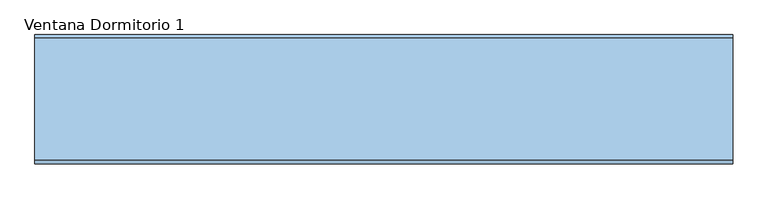
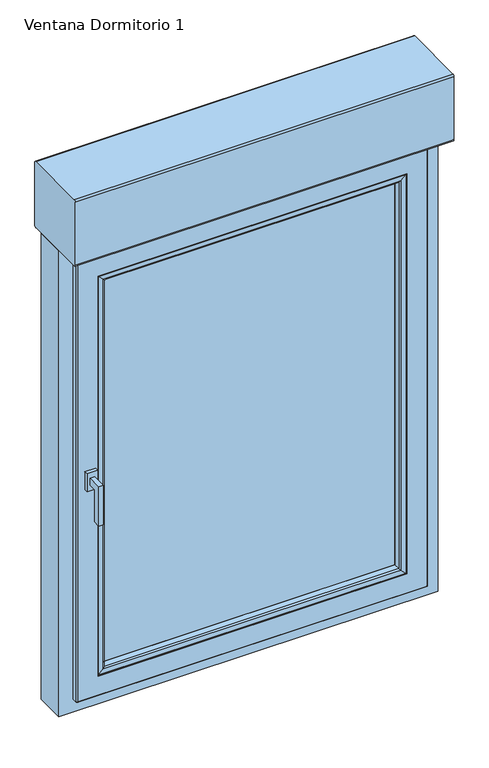
"""IFC4 building model written with IfcOpenShell, lengths in millimetres: window geometry, 2019_ES_Ventana_Replus_re80pvc301_10100_box_1-Hoja_con-Compacto : Ventana Dormitorio 1."""

from ifc_helpers import new_model, si_unit, point, frame, frame_2d, origin, place, context, project, spatial, polyline, circle_curve, ellipse_curve, trimmed, segment, composite_curve, outline, extrude, source, transform, mapped, element, save
from ifc_brep_helpers import plane_surface, cylinder_surface, advanced_brep


def ventana_dormitorio_1_e636b9de(model_context):
    return source(origin(), model_context, "Body", "SolidModel", [
        extrude(outline(composite_curve([segment(polyline([(55.0, 2110.0), (-120.0, 2110.0)]), True, "CONTINUOUS"), segment(trimmed(circle_curve(frame_2d((-120.0, 2115.0)), 5.0), [point((-120.0, 2110.0))], [point((-125.0, 2115.0))], False, "CARTESIAN"), True, "CONTINUOUS"), segment(polyline([(-125.0, 2115.0), (-125.0, 2290.0)]), True, "CONTINUOUS"), segment(trimmed(circle_curve(frame_2d((-120.0, 2290.0)), 5.0), [point((-125.0, 2290.0))], [point((-120.0, 2295.0))], False, "CARTESIAN"), True, "CONTINUOUS"), segment(polyline([(-120.0, 2295.0), (55.0, 2295.0)]), True, "CONTINUOUS"), segment(trimmed(circle_curve(frame_2d((55.0, 2290.0)), 5.0), [point((55.0, 2295.0))], [point((60.0, 2290.0))], False, "CARTESIAN"), True, "CONTINUOUS"), segment(polyline([(60.0, 2290.0), (60.0, 2115.0)]), True, "CONTINUOUS"), segment(trimmed(circle_curve(frame_2d((55.0, 2115.0)), 5.0), [point((60.0, 2115.0))], [point((55.0, 2110.0))], False, "CARTESIAN"), True, "CONTINUOUS")], self_intersect=False)), frame((-500.0, 0.0, 0.0), z_axis=(1.0, 0.0, 0.0), x_axis=(0.0, 1.0, 0.0)), (0.0, 0.0, 1.0), 1000.0),
        extrude(outline(polyline([(-78.4999991, 1470.0), (-78.4999991, 1450.0), (-98.4999991, 1450.0), (-98.4999991, 1360.0), (-118.4999991, 1360.0), (-118.4999991, 1470.0), (-78.4999991, 1470.0)])), frame((-434.1999993, 0.0, 0.0), z_axis=(1.0, 0.0, 0.0), x_axis=(0.0, 1.0, 0.0)), (0.0, 0.0, 1.0), 12.0),
        extrude(outline(polyline([(-413.9687607, -78.4999991), (-442.4312378, -78.4999991), (-442.4312378, -68.4999991), (-413.9687607, -68.4999991), (-413.9687607, -78.4999991)])), frame((0.0, 0.0, 1435.217127), z_axis=(0.0, 0.0, 1.0), x_axis=(1.0, 0.0, 0.0)), (0.0, 0.0, 1.0), 49.565746),
        extrude(outline(polyline([(2007.2, 397.1999993), (2007.2, -397.1999993), (909.8, -397.1999993), (909.8, 397.1999993), (2007.2, 397.1999993)]), holes=[polyline([(917.8, 389.1999993), (917.8, -389.1999993), (1999.2, -389.1999993), (1999.2, 389.1999993), (917.8, 389.1999993)])]), frame((0.0, -26.9999999, 0.0), z_axis=(0.0, 1.0, 0.0), x_axis=(0.0, 0.0, 1.0)), (0.0, 0.0, 1.0), 16.0),
        extrude(outline(polyline([(2007.1868066, 397.1868058), (2007.1868066, -397.1868058), (909.8131934, -397.1868058), (909.8131934, 397.1868058), (2007.1868066, 397.1868058)]), holes=[polyline([(917.8, 389.1999993), (917.8, -389.1999993), (1999.2, -389.1999993), (1999.2, 389.1999993), (917.8, 389.1999993)])]), frame((0.0, -47.0000001, 0.0), z_axis=(0.0, 1.0, 0.0), x_axis=(0.0, 0.0, 1.0)), (0.0, 0.0, 1.0), 16.0),
        extrude(outline(polyline([(397.1999993, -6.9999997), (397.1999993, -10.9999999), (-397.1999993, -10.9999999), (-397.1999993, -6.9999997), (397.1999993, -6.9999997)])), frame((0.0, 0.0, 903.7946451), z_axis=(0.0, 0.0, 1.0), x_axis=(1.0, 0.0, 0.0)), (0.0, 0.0, 1.0), 1109.4053549),
        extrude(outline(polyline([(397.1999993, -26.9999999), (397.1999993, -31.0000001), (-397.1999993, -31.0000001), (-397.1999993, -26.9999999), (397.1999993, -26.9999999)])), frame((0.0, 0.0, 903.7946451), z_axis=(0.0, 0.0, 1.0), x_axis=(1.0, 0.0, 0.0)), (0.0, 0.0, 1.0), 1109.4053549),
        extrude(outline(polyline([(397.1999993, -47.0000001), (397.1999993, -51.0000003), (-397.1999993, -51.0000003), (-397.1999993, -47.0000001), (397.1999993, -47.0000001)])), frame((0.0, 0.0, 903.7946451), z_axis=(0.0, 0.0, 1.0), x_axis=(1.0, 0.0, 0.0)), (0.0, 0.0, 1.0), 1109.4053549),
        advanced_brep(
        [(387.2913171, 9.2764571, 1997.2913178), (390.1890946, 11.5, 2000.1890953), (390.1890946, 11.5, 919.8109047), (387.2913171, 9.2764571, 922.7086822), (430.1999993, 11.5, 879.8), (-430.1999993, 11.5, 879.8), (-430.1999993, 11.5, 2040.2), (430.1999993, 11.5, 2040.2), (-390.1890946, 11.5, 2000.1890953), (-390.1890946, 11.5, 919.8109047), (-387.2913171, 9.2764571, 922.7086822), (384.1757968, -2.3508228, 1994.1757976), (384.1757968, -2.3508228, 925.8242024), (-384.1757968, -2.3508228, 925.8242024), (384.6739305, -3.0000033, 1994.6739313), (384.6739305, -3.0000033, 925.3260687), (-384.6739305, -3.0000033, 925.3260687), (391.1999993, -3.0000033, 2001.2), (-391.1999993, -3.0000033, 2001.2), (-391.1999993, -3.0000033, 918.8), (391.1999993, -3.0000033, 918.8), (-384.6739305, -3.0000033, 1994.6739313), (391.1999993, -6.9999997, 2001.2), (391.1999993, -6.9999997, 918.8), (-391.1999993, -6.9999997, 918.8), (411.8162192, -6.9999997, 2021.8162199), (-411.8162192, -6.9999997, 2021.8162199), (-411.8162192, -6.9999997, 898.1837801), (411.8162192, -6.9999997, 898.1837801), (-391.1999993, -6.9999997, 2001.2), (409.1999993, -25.6153717, 2019.2), (409.1999993, -25.6153717, 900.8), (-409.1999993, -25.6153717, 900.8), (409.1999993, -56.4999995, 2019.2), (409.1999993, -56.4999995, 900.8), (-409.1999993, -56.4999995, 900.8), (-409.1999993, -56.4999995, 2019.2), (397.1999993, -56.4999995, 2007.2), (-397.1999993, -56.4999995, 2007.2), (-397.1999993, -56.4999995, 912.8), (397.1999993, -56.4999995, 912.8), (397.1999993, -51.0000003, 2007.2), (397.1999993, -51.0000003, 912.8), (-397.1999993, -51.0000003, 912.8), (-397.1999993, -51.0000003, 2007.2), (386.007687, -51.0000003, 1996.0076877), (-386.007687, -51.0000003, 1996.0076877), (-386.007687, -51.0000003, 923.9923123), (386.007687, -51.0000003, 923.9923123), (385.4940999, -51.6693201, 1995.4941006), (385.4940999, -51.6693201, 924.5058994), (-385.4940999, -51.6693201, 924.5058994), (388.8993918, -64.3780426, 1998.8993925), (388.8993918, -64.3780426, 921.1006075), (-388.8993918, -64.3780426, 921.1006075), (392.6234971, -67.3403297, 2002.6234978), (392.6234971, -67.3403297, 917.3765022), (-392.6234971, -67.3403297, 917.3765022), (405.6488427, -67.7951848, 2015.6488434), (405.6488427, -67.7951848, 904.3511566), (-405.6488427, -67.7951848, 904.3511566), (406.1999993, -67.2629391, 2016.2), (406.1999993, -67.2629391, 903.8), (-406.1999993, -67.2629391, 903.8), (407.4370593, -68.4999991, 2017.43706), (407.4370593, -68.4999991, 902.56294), (-407.4370593, -68.4999991, 902.56294), (460.1999993, -68.4999991, 2070.2), (-460.1999993, -68.4999991, 2070.2), (-460.1999993, -68.4999991, 849.8), (460.1999993, -68.4999991, 849.8), (-407.4370593, -68.4999991, 2017.43706), (463.1999993, -65.4999991, 2073.2), (463.1999993, -65.4999991, 846.8), (-463.1999993, -65.4999991, 846.8), (463.1999993, -50.0, 2073.2), (463.1999993, -50.0, 846.8), (-463.1999993, -50.0, 846.8), (-463.1999993, -50.0, 2073.2), (443.1999993, -50.0, 2053.2), (-443.1999993, -50.0, 2053.2), (-443.1999993, -50.0, 866.8), (443.1999993, -50.0, 866.8), (443.1999993, -11.9999991, 866.8), (443.1999993, -11.9999991, 2053.2), (-443.1999993, -11.9999991, 866.8), (-443.1999993, -11.9999991, 2053.2), (430.1999993, -11.9999991, 2040.2), (-430.1999993, -11.9999991, 2040.2), (-430.1999993, -11.9999991, 879.8), (430.1999993, -11.9999991, 879.8), (-387.2913171, 9.2764571, 1997.2913178), (-384.1757968, -2.3508228, 1994.1757976), (-409.1999993, -25.6153717, 2019.2), (-385.4940999, -51.6693201, 1995.4941006), (-388.8993918, -64.3780426, 1998.8993925), (-392.6234971, -67.3403297, 2002.6234978), (-405.6488427, -67.7951848, 2015.6488434), (-406.1999993, -67.2629391, 2016.2), (-463.1999993, -65.4999991, 2073.2)],
        [
            (0, 1, ellipse_curve(frame((390.1890946, 8.5, 2000.1890953), z_axis=(0.7071067811865475, 0.0, -0.7071067811865475), x_axis=(0.7071067811865474, 0.0, 0.7071067811865476)), 4.2426407, 3.0)),
            (1, 2),
            (2, 3, ellipse_curve(frame((390.1890946, 8.5, 919.8109047), z_axis=(0.7071067811865475, 0.0, 0.7071067811865475), x_axis=(-0.7071067811865474, 0.0, 0.7071067811865476)), 4.2426407, 3.0)),
            (3, 0),
            (4, 5),
            (5, 6),
            (6, 7),
            (7, 4),
            (1, 8),
            (8, 9),
            (9, 2),
            (9, 10, ellipse_curve(frame((-390.1890946, 8.5, 919.8109047), z_axis=(0.7071067811865475, 0.0, -0.7071067811865475), x_axis=(0.7071067811865476, 0.0, 0.7071067811865474)), 4.2426407, 3.0)),
            (10, 3),
            (11, 0),
            (3, 12),
            (12, 11),
            (10, 13),
            (13, 12),
            (14, 11, ellipse_curve(frame((384.6739305, -2.4842973, 1994.6739313), z_axis=(0.7071067811865475, 0.0, -0.7071067811865475), x_axis=(0.7071067811865474, 0.0, 0.7071067811865476)), 0.7293184, 0.515706)),
            (12, 15, ellipse_curve(frame((384.6739305, -2.4842973, 925.3260687), z_axis=(0.7071067811865475, 0.0, 0.7071067811865475), x_axis=(-0.7071067811865474, 0.0, 0.7071067811865476)), 0.7293184, 0.515706)),
            (15, 14),
            (13, 16, ellipse_curve(frame((-384.6739305, -2.4842973, 925.3260687), z_axis=(0.7071067811865475, 0.0, -0.7071067811865475), x_axis=(0.7071067811865476, 0.0, 0.7071067811865474)), 0.7293184, 0.515706)),
            (16, 15),
            (17, 18),
            (18, 19),
            (19, 20),
            (20, 17),
            (16, 21),
            (21, 14),
            (22, 17),
            (20, 23),
            (23, 22),
            (19, 24),
            (24, 23),
            (25, 26),
            (26, 27),
            (27, 28),
            (28, 25),
            (24, 29),
            (29, 22),
            (30, 25),
            (28, 31),
            (31, 30),
            (27, 32),
            (32, 31),
            (33, 30),
            (31, 34),
            (34, 33),
            (32, 35),
            (35, 34),
            (35, 36),
            (36, 33),
            (37, 38),
            (38, 39),
            (39, 40),
            (40, 37),
            (41, 37),
            (40, 42),
            (42, 41),
            (39, 43),
            (43, 42),
            (43, 44),
            (44, 41),
            (45, 46),
            (46, 47),
            (47, 48),
            (48, 45),
            (49, 45, ellipse_curve(frame((386.007687, -51.5317048, 1996.0076877), z_axis=(0.7071067811865475, 0.0, -0.7071067811865475), x_axis=(0.7071067811865474, 0.0, 0.7071067811865476)), 0.7519437, 0.5317045)),
            (48, 50, ellipse_curve(frame((386.007687, -51.5317048, 923.9923123), z_axis=(0.7071067811865475, 0.0, 0.7071067811865475), x_axis=(-0.7071067811865474, 0.0, 0.7071067811865476)), 0.7519437, 0.5317045)),
            (50, 49),
            (47, 51, ellipse_curve(frame((-386.007687, -51.5317048, 923.9923123), z_axis=(0.7071067811865475, 0.0, -0.7071067811865475), x_axis=(0.7071067811865476, 0.0, 0.7071067811865474)), 0.7519437, 0.5317045)),
            (51, 50),
            (52, 49),
            (50, 53),
            (53, 52),
            (51, 54),
            (54, 53),
            (55, 52, ellipse_curve(frame((392.7630951, -63.3427664, 2002.7630958), z_axis=(0.7071067811865475, 0.0, -0.7071067811865475), x_axis=(0.7071067811865474, 0.0, 0.7071067811865476)), 5.6568542, 4.0)),
            (53, 56, ellipse_curve(frame((392.7630951, -63.3427664, 917.2369042), z_axis=(0.7071067811865475, 0.0, 0.7071067811865475), x_axis=(-0.7071067811865474, 0.0, 0.7071067811865476)), 5.6568542, 4.0)),
            (56, 55),
            (54, 57, ellipse_curve(frame((-392.7630951, -63.3427664, 917.2369042), z_axis=(0.7071067811865475, 0.0, -0.7071067811865475), x_axis=(0.7071067811865476, 0.0, 0.7071067811865474)), 5.6568542, 4.0)),
            (57, 56),
            (58, 55),
            (56, 59),
            (59, 58),
            (57, 60),
            (60, 59),
            (61, 58, ellipse_curve(frame((405.6674291, -67.2629391, 2015.6674299), z_axis=(0.7071067811865475, 0.0, -0.7071067811865475), x_axis=(0.7071067811865474, 0.0, 0.7071067811865476)), 0.7531679, 0.5325701)),
            (59, 62, ellipse_curve(frame((405.6674291, -67.2629391, 904.3325701), z_axis=(0.7071067811865475, 0.0, 0.7071067811865475), x_axis=(-0.7071067811865474, 0.0, 0.7071067811865476)), 0.7531679, 0.5325701)),
            (62, 61),
            (60, 63, ellipse_curve(frame((-405.6674291, -67.2629391, 904.3325701), z_axis=(0.7071067811865475, 0.0, -0.7071067811865475), x_axis=(0.7071067811865476, 0.0, 0.7071067811865474)), 0.7531679, 0.5325701)),
            (63, 62),
            (64, 61, ellipse_curve(frame((407.4370593, -67.2629391, 2017.43706), z_axis=(0.7071067811865475, 0.0, -0.7071067811865475), x_axis=(0.7071067811865474, 0.0, 0.7071067811865476)), 1.7494671, 1.23706)),
            (62, 65, ellipse_curve(frame((407.4370593, -67.2629391, 902.56294), z_axis=(0.7071067811865475, 0.0, 0.7071067811865475), x_axis=(-0.7071067811865474, 0.0, 0.7071067811865476)), 1.7494671, 1.23706)),
            (65, 64),
            (63, 66, ellipse_curve(frame((-407.4370593, -67.2629391, 902.56294), z_axis=(0.7071067811865475, 0.0, -0.7071067811865475), x_axis=(0.7071067811865476, 0.0, 0.7071067811865474)), 1.7494671, 1.23706)),
            (66, 65),
            (67, 68),
            (68, 69),
            (69, 70),
            (70, 67),
            (66, 71),
            (71, 64),
            (72, 67, ellipse_curve(frame((460.1999993, -65.4999991, 2070.2), z_axis=(0.7071067811865475, 0.0, -0.7071067811865475), x_axis=(0.7071067811865474, 0.0, 0.7071067811865476)), 4.2426407, 3.0)),
            (70, 73, ellipse_curve(frame((460.1999993, -65.4999991, 849.8), z_axis=(0.7071067811865475, 0.0, 0.7071067811865475), x_axis=(-0.7071067811865474, 0.0, 0.7071067811865476)), 4.2426407, 3.0)),
            (73, 72),
            (69, 74, ellipse_curve(frame((-460.1999993, -65.4999991, 849.8), z_axis=(0.7071067811865475, 0.0, -0.7071067811865475), x_axis=(0.7071067811865476, 0.0, 0.7071067811865474)), 4.2426407, 3.0)),
            (74, 73),
            (75, 72),
            (73, 76),
            (76, 75),
            (74, 77),
            (77, 76),
            (77, 78),
            (78, 75),
            (79, 80),
            (80, 81),
            (81, 82),
            (82, 79),
            (82, 83),
            (83, 84),
            (84, 79),
            (81, 85),
            (85, 83),
            (85, 86),
            (86, 84),
            (87, 88),
            (88, 89),
            (89, 90),
            (90, 87),
            (90, 4),
            (7, 87),
            (89, 5),
            (8, 91, ellipse_curve(frame((-390.1890946, 8.5, 2000.1890953), z_axis=(-0.7071067811865475, 0.0, -0.7071067811865475), x_axis=(0.7071067811865474, 0.0, -0.7071067811865476)), 4.2426407, 3.0)),
            (91, 10),
            (91, 92),
            (92, 13),
            (92, 21, ellipse_curve(frame((-384.6739305, -2.4842973, 1994.6739313), z_axis=(-0.7071067811865475, 0.0, -0.7071067811865475), x_axis=(0.7071067811865474, 0.0, -0.7071067811865476)), 0.7293184, 0.515706)),
            (18, 29),
            (26, 93),
            (93, 32),
            (93, 36),
            (38, 44),
            (46, 94, ellipse_curve(frame((-386.007687, -51.5317048, 1996.0076877), z_axis=(-0.7071067811865475, 0.0, -0.7071067811865475), x_axis=(0.7071067811865474, 0.0, -0.7071067811865476)), 0.7519437, 0.5317045)),
            (94, 51),
            (94, 95),
            (95, 54),
            (95, 96, ellipse_curve(frame((-392.7630951, -63.3427664, 2002.7630958), z_axis=(-0.7071067811865475, 0.0, -0.7071067811865475), x_axis=(0.7071067811865474, 0.0, -0.7071067811865476)), 5.6568542, 4.0)),
            (96, 57),
            (96, 97),
            (97, 60),
            (97, 98, ellipse_curve(frame((-405.6674291, -67.2629391, 2015.6674299), z_axis=(-0.7071067811865475, 0.0, -0.7071067811865475), x_axis=(0.7071067811865474, 0.0, -0.7071067811865476)), 0.7531679, 0.5325701)),
            (98, 63),
            (98, 71, ellipse_curve(frame((-407.4370593, -67.2629391, 2017.43706), z_axis=(-0.7071067811865475, 0.0, -0.7071067811865475), x_axis=(0.7071067811865474, 0.0, -0.7071067811865476)), 1.7494671, 1.23706)),
            (68, 99, ellipse_curve(frame((-460.1999993, -65.4999991, 2070.2), z_axis=(-0.7071067811865475, 0.0, -0.7071067811865475), x_axis=(0.7071067811865474, 0.0, -0.7071067811865476)), 4.2426407, 3.0)),
            (99, 74),
            (99, 78),
            (80, 86),
            (88, 6),
            (0, 91),
            (11, 92),
            (30, 93),
            (49, 94),
            (52, 95),
            (55, 96),
            (58, 97),
            (61, 98),
            (72, 99),
        ],
        [
            cylinder_surface(frame((390.1890946, 8.5, 2073.2), z_axis=(0.0, 0.0, 1.0), x_axis=(-1.0, 0.0, 0.0)), 3.0),
            plane_surface(frame((-430.1999993, 11.5, 2040.2), z_axis=(0.0, 1.0, 0.0), x_axis=(1.0, 0.0, 0.0))),
            cylinder_surface(frame((463.1999993, 8.5, 919.8109047), z_axis=(1.0, 0.0, 0.0), x_axis=(0.0, 0.0, 1.0)), 3.0),
            plane_surface(frame((387.2913171, 9.2764571, 1997.2913178), z_axis=(-0.9659258263570549, 0.2588190448487916, 0.0), x_axis=(0.0, 0.0, -1.0))),
            plane_surface(frame((387.2913171, 9.2764571, 922.7086822), z_axis=(0.0, 0.2588190448487885, 0.9659258263570558), x_axis=(-1.0, 0.0, 0.0))),
            cylinder_surface(frame((384.6739305, -2.4842973, 2073.2), z_axis=(0.0, 0.0, 1.0), x_axis=(-1.0, 0.0, 0.0)), 0.515706),
            cylinder_surface(frame((463.1999993, -2.4842973, 925.3260687), z_axis=(1.0, 0.0, 0.0), x_axis=(0.0, 0.0, 1.0)), 0.515706),
            plane_surface(frame((-384.6739305, -3.0000033, 1994.6739313), z_axis=(0.0, -1.0, 0.0), x_axis=(1.0, 0.0, 0.0))),
            plane_surface(frame((391.1999993, -3.0000033, 2001.2), z_axis=(-1.0, 0.0, 0.0), x_axis=(0.0, 0.0, -1.0))),
            plane_surface(frame((391.1999993, -3.0000033, 918.8), z_axis=(0.0, 0.0, 1.0), x_axis=(-1.0, 0.0, 0.0))),
            plane_surface(frame((-391.1999993, -6.9999997, 2001.2), z_axis=(0.0, -1.0, 0.0), x_axis=(1.0, 0.0, 0.0))),
            plane_surface(frame((411.8162192, -6.9999997, 2021.8162199), z_axis=(-0.9902680687415736, 0.13917310096004265, 0.0), x_axis=(0.0, 0.0, -1.0))),
            plane_surface(frame((411.8162192, -6.9999997, 898.1837801), z_axis=(0.0, 0.13917310096003946, 0.990268068741574), x_axis=(-1.0, 0.0, 0.0))),
            plane_surface(frame((409.1999993, -25.6153717, 2019.2), z_axis=(-1.0, 0.0, 0.0), x_axis=(0.0, 0.0, -1.0))),
            plane_surface(frame((409.1999993, -25.6153717, 900.8), z_axis=(0.0, 0.0, 1.0), x_axis=(-1.0, 0.0, 0.0))),
            plane_surface(frame((-409.1999993, -56.4999995, 2019.2), z_axis=(0.0, 1.0, 0.0), x_axis=(1.0, 0.0, 0.0))),
            plane_surface(frame((397.1999993, -56.4999995, 2007.2), z_axis=(1.0, 0.0, 0.0), x_axis=(0.0, 0.0, -1.0))),
            plane_surface(frame((397.1999993, -56.4999995, 912.8), z_axis=(0.0, 0.0, -1.0), x_axis=(-1.0, 0.0, 0.0))),
            plane_surface(frame((-397.1999993, -51.0000003, 2007.2), z_axis=(0.0, 1.0, 0.0), x_axis=(1.0, 0.0, 0.0))),
            cylinder_surface(frame((386.007687, -51.5317048, 2073.2), z_axis=(0.0, 0.0, 1.0), x_axis=(-1.0, 0.0, 0.0)), 0.5317045),
            cylinder_surface(frame((463.1999993, -51.5317048, 923.9923123), z_axis=(1.0, 0.0, 0.0), x_axis=(0.0, 0.0, 1.0)), 0.5317045),
            plane_surface(frame((385.4940999, -51.6693201, 1995.4941006), z_axis=(-0.9659258262890666, -0.2588190451025272, 0.0), x_axis=(0.0, 0.0, -1.0))),
            plane_surface(frame((385.4940999, -51.6693201, 924.5058994), z_axis=(0.0, -0.2588190451025303, 0.9659258262890658), x_axis=(-1.0, 0.0, 0.0))),
            cylinder_surface(frame((392.7630951, -63.3427664, 2073.2), z_axis=(0.0, 0.0, 1.0), x_axis=(-1.0, 0.0, 0.0)), 4.0),
            cylinder_surface(frame((463.1999993, -63.3427664, 917.2369042), z_axis=(1.0, 0.0, 0.0), x_axis=(0.0, 0.0, 1.0)), 4.0),
            plane_surface(frame((392.6234971, -67.3403297, 2002.6234978), z_axis=(-0.034899496702507804, -0.9993908270190955, 0.0), x_axis=(0.0, 0.0, -1.0))),
            plane_surface(frame((392.6234971, -67.3403297, 917.3765022), z_axis=(0.0, -0.9993908270190957, 0.03489949670250457), x_axis=(-1.0, 0.0, 0.0))),
            cylinder_surface(frame((405.6674291, -67.2629391, 2073.2), z_axis=(0.0, 0.0, 1.0), x_axis=(-1.0, 0.0, 0.0)), 0.5325701),
            cylinder_surface(frame((463.1999993, -67.2629391, 904.3325701), z_axis=(1.0, 0.0, 0.0), x_axis=(0.0, 0.0, 1.0)), 0.5325701),
            cylinder_surface(frame((407.4370593, -67.2629391, 2073.2), z_axis=(0.0, 0.0, 1.0), x_axis=(-1.0, 0.0, 0.0)), 1.23706),
            cylinder_surface(frame((463.1999993, -67.2629391, 902.56294), z_axis=(1.0, 0.0, 0.0), x_axis=(0.0, 0.0, 1.0)), 1.23706),
            plane_surface(frame((-407.4370593, -68.4999991, 2017.43706), z_axis=(0.0, -1.0, 0.0), x_axis=(1.0, 0.0, 0.0))),
            cylinder_surface(frame((460.1999993, -65.4999991, 2073.2), z_axis=(0.0, 0.0, 1.0), x_axis=(-1.0, 0.0, 0.0)), 3.0),
            cylinder_surface(frame((463.1999993, -65.4999991, 849.8), z_axis=(1.0, 0.0, 0.0), x_axis=(0.0, 0.0, 1.0)), 3.0),
            plane_surface(frame((463.1999993, -65.4999991, 2073.2), z_axis=(1.0, 0.0, 0.0), x_axis=(0.0, 0.0, -1.0))),
            plane_surface(frame((463.1999993, -65.4999991, 846.8), z_axis=(0.0, 0.0, -1.0), x_axis=(-1.0, 0.0, 0.0))),
            plane_surface(frame((-459.2000019, -50.0, 2069.2000027), z_axis=(0.0, 1.0, 0.0), x_axis=(1.0, 0.0, 0.0))),
            plane_surface(frame((443.1999993, -45.0999991, 2053.2), z_axis=(1.0, 0.0, 0.0), x_axis=(0.0, 0.0, -1.0))),
            plane_surface(frame((443.1999993, -45.0999991, 866.8), z_axis=(0.0, 0.0, -1.0), x_axis=(-1.0, 0.0, 0.0))),
            plane_surface(frame((-435.7000002, -11.9999991, 2045.7000009), z_axis=(0.0, 1.0, 0.0), x_axis=(1.0, 0.0, 0.0))),
            plane_surface(frame((430.1999993, -1.4999991, 2040.2), z_axis=(1.0, 0.0, 0.0), x_axis=(0.0, 0.0, -1.0))),
            plane_surface(frame((430.1999993, -1.4999991, 879.8), z_axis=(0.0, 0.0, -1.0), x_axis=(-1.0, 0.0, 0.0))),
            cylinder_surface(frame((-390.1890946, 8.5, 846.8), z_axis=(0.0, 0.0, -1.0), x_axis=(1.0, 0.0, 0.0)), 3.0),
            plane_surface(frame((-387.2913171, 9.2764571, 922.7086822), z_axis=(0.9659258263570565, 0.2588190448487853, 0.0), x_axis=(0.0, 0.0, 1.0))),
            cylinder_surface(frame((-384.6739305, -2.4842973, 846.8), z_axis=(0.0, 0.0, -1.0), x_axis=(1.0, 0.0, 0.0)), 0.515706),
            plane_surface(frame((-391.1999993, -3.0000033, 918.8), z_axis=(1.0, 0.0, 0.0), x_axis=(0.0, 0.0, 1.0))),
            plane_surface(frame((-411.8162192, -6.9999997, 898.1837801), z_axis=(0.9902680687415745, 0.13917310096003627, 0.0), x_axis=(0.0, 0.0, 1.0))),
            plane_surface(frame((-409.1999993, -25.6153717, 900.8), z_axis=(1.0, 0.0, 0.0), x_axis=(0.0, 0.0, 1.0))),
            plane_surface(frame((-397.1999993, -56.4999995, 912.8), z_axis=(-1.0, 0.0, 0.0), x_axis=(0.0, 0.0, 1.0))),
            cylinder_surface(frame((-386.007687, -51.5317048, 846.8), z_axis=(0.0, 0.0, -1.0), x_axis=(1.0, 0.0, 0.0)), 0.5317045),
            plane_surface(frame((-385.4940999, -51.6693201, 924.5058994), z_axis=(0.9659258262890649, -0.2588190451025334, 0.0), x_axis=(0.0, 0.0, 1.0))),
            cylinder_surface(frame((-392.7630951, -63.3427664, 846.8), z_axis=(0.0, 0.0, -1.0), x_axis=(1.0, 0.0, 0.0)), 4.0),
            plane_surface(frame((-392.6234971, -67.3403297, 917.3765022), z_axis=(0.03489949670250134, -0.9993908270190958, 0.0), x_axis=(0.0, 0.0, 1.0))),
            cylinder_surface(frame((-405.6674291, -67.2629391, 846.8), z_axis=(0.0, 0.0, -1.0), x_axis=(1.0, 0.0, 0.0)), 0.5325701),
            cylinder_surface(frame((-407.4370593, -67.2629391, 846.8), z_axis=(0.0, 0.0, -1.0), x_axis=(1.0, 0.0, 0.0)), 1.23706),
            cylinder_surface(frame((-460.1999993, -65.4999991, 846.8), z_axis=(0.0, 0.0, -1.0), x_axis=(1.0, 0.0, 0.0)), 3.0),
            plane_surface(frame((-463.1999993, -65.4999991, 846.8), z_axis=(-1.0, 0.0, 0.0), x_axis=(0.0, 0.0, 1.0))),
            plane_surface(frame((-443.1999993, -45.0999991, 866.8), z_axis=(-1.0, 0.0, 0.0), x_axis=(0.0, 0.0, 1.0))),
            plane_surface(frame((-430.1999993, -1.4999991, 879.8), z_axis=(-1.0, 0.0, 0.0), x_axis=(0.0, 0.0, 1.0))),
            cylinder_surface(frame((-463.1999993, 8.5, 2000.1890953), z_axis=(-1.0, 0.0, 0.0), x_axis=(0.0, 0.0, -1.0)), 3.0),
            plane_surface(frame((-387.2913171, 9.2764571, 1997.2913178), z_axis=(0.0, 0.2588190448487885, -0.9659258263570557), x_axis=(1.0, 0.0, 0.0))),
            cylinder_surface(frame((-463.1999993, -2.4842973, 1994.6739313), z_axis=(-1.0, 0.0, 0.0), x_axis=(0.0, 0.0, -1.0)), 0.515706),
            plane_surface(frame((-391.1999993, -3.0000033, 2001.2), z_axis=(0.0, 0.0, -1.0), x_axis=(1.0, 0.0, 0.0))),
            plane_surface(frame((-411.8162192, -6.9999997, 2021.8162199), z_axis=(0.0, 0.13917310096003946, -0.990268068741574), x_axis=(1.0, 0.0, 0.0))),
            plane_surface(frame((-409.1999993, -25.6153717, 2019.2), z_axis=(0.0, 0.0, -1.0), x_axis=(1.0, 0.0, 0.0))),
            plane_surface(frame((-397.1999993, -56.4999995, 2007.2), z_axis=(0.0, 0.0, 1.0), x_axis=(1.0, 0.0, 0.0))),
            cylinder_surface(frame((-463.1999993, -51.5317048, 1996.0076877), z_axis=(-1.0, 0.0, 0.0), x_axis=(0.0, 0.0, -1.0)), 0.5317045),
            plane_surface(frame((-385.4940999, -51.6693201, 1995.4941006), z_axis=(0.0, -0.2588190451025303, -0.9659258262890658), x_axis=(1.0, 0.0, 0.0))),
            cylinder_surface(frame((-463.1999993, -63.3427664, 2002.7630958), z_axis=(-1.0, 0.0, 0.0), x_axis=(0.0, 0.0, -1.0)), 4.0),
            plane_surface(frame((-392.6234971, -67.3403297, 2002.6234978), z_axis=(0.0, -0.9993908270190957, -0.03489949670250457), x_axis=(1.0, 0.0, 0.0))),
            cylinder_surface(frame((-463.1999993, -67.2629391, 2015.6674299), z_axis=(-1.0, 0.0, 0.0), x_axis=(0.0, 0.0, -1.0)), 0.5325701),
            cylinder_surface(frame((-463.1999993, -67.2629391, 2017.43706), z_axis=(-1.0, 0.0, 0.0), x_axis=(0.0, 0.0, -1.0)), 1.23706),
            cylinder_surface(frame((-463.1999993, -65.4999991, 2070.2), z_axis=(-1.0, 0.0, 0.0), x_axis=(0.0, 0.0, -1.0)), 3.0),
            plane_surface(frame((-463.1999993, -65.4999991, 2073.2), z_axis=(0.0, 0.0, 1.0), x_axis=(1.0, 0.0, 0.0))),
            plane_surface(frame((-443.1999993, -45.0999991, 2053.2), z_axis=(0.0, 0.0, 1.0), x_axis=(1.0, 0.0, 0.0))),
            plane_surface(frame((-430.1999993, -1.4999991, 2040.2), z_axis=(0.0, 0.0, 1.0), x_axis=(1.0, 0.0, 0.0))),
        ],
        [
            (0, [[1, 2, 3, 4]]),
            (1, [[5, 6, 7, 8], [9, 10, 11, -2]]),
            (2, [[-3, -11, 12, 13]]),
            (3, [[14, -4, 15, 16]]),
            (4, [[-15, -13, 17, 18]]),
            (5, [[19, -16, 20, 21]]),
            (6, [[-20, -18, 22, 23]]),
            (7, [[24, 25, 26, 27], [-23, 28, 29, -21]]),
            (8, [[30, -27, 31, 32]]),
            (9, [[-31, -26, 33, 34]]),
            (10, [[35, 36, 37, 38], [-34, 39, 40, -32]]),
            (11, [[41, -38, 42, 43]]),
            (12, [[-42, -37, 44, 45]]),
            (13, [[46, -43, 47, 48]]),
            (14, [[-47, -45, 49, 50]]),
            (15, [[-50, 51, 52, -48], [53, 54, 55, 56]]),
            (16, [[57, -56, 58, 59]]),
            (17, [[-58, -55, 60, 61]]),
            (18, [[-61, 62, 63, -59], [64, 65, 66, 67]]),
            (19, [[68, -67, 69, 70]]),
            (20, [[-69, -66, 71, 72]]),
            (21, [[73, -70, 74, 75]]),
            (22, [[-74, -72, 76, 77]]),
            (23, [[78, -75, 79, 80]]),
            (24, [[-79, -77, 81, 82]]),
            (25, [[83, -80, 84, 85]]),
            (26, [[-84, -82, 86, 87]]),
            (27, [[88, -85, 89, 90]]),
            (28, [[-89, -87, 91, 92]]),
            (29, [[93, -90, 94, 95]]),
            (30, [[-94, -92, 96, 97]]),
            (31, [[98, 99, 100, 101], [-97, 102, 103, -95]]),
            (32, [[104, -101, 105, 106]]),
            (33, [[-105, -100, 107, 108]]),
            (34, [[109, -106, 110, 111]]),
            (35, [[-110, -108, 112, 113]]),
            (36, [[-113, 114, 115, -111], [116, 117, 118, 119]]),
            (37, [[-119, 120, 121, 122]]),
            (38, [[-120, -118, 123, 124]]),
            (39, [[-124, 125, 126, -121], [127, 128, 129, 130]]),
            (40, [[-130, 131, -8, 132]]),
            (41, [[-131, -129, 133, -5]]),
            (42, [[-12, -10, 134, 135]]),
            (43, [[-17, -135, 136, 137]]),
            (44, [[-22, -137, 138, -28]]),
            (45, [[-33, -25, 139, -39]]),
            (46, [[-44, -36, 140, 141]]),
            (47, [[-49, -141, 142, -51]]),
            (48, [[-60, -54, 143, -62]]),
            (49, [[-71, -65, 144, 145]]),
            (50, [[-76, -145, 146, 147]]),
            (51, [[-81, -147, 148, 149]]),
            (52, [[-86, -149, 150, 151]]),
            (53, [[-91, -151, 152, 153]]),
            (54, [[-96, -153, 154, -102]]),
            (55, [[-107, -99, 155, 156]]),
            (56, [[-112, -156, 157, -114]]),
            (57, [[-123, -117, 158, -125]]),
            (58, [[-133, -128, 159, -6]]),
            (59, [[-134, -9, -1, 160]]),
            (60, [[-136, -160, -14, 161]]),
            (61, [[-138, -161, -19, -29]]),
            (62, [[-139, -24, -30, -40]]),
            (63, [[-140, -35, -41, 162]]),
            (64, [[-142, -162, -46, -52]]),
            (65, [[-143, -53, -57, -63]]),
            (66, [[-144, -64, -68, 163]]),
            (67, [[-146, -163, -73, 164]]),
            (68, [[-148, -164, -78, 165]]),
            (69, [[-150, -165, -83, 166]]),
            (70, [[-152, -166, -88, 167]]),
            (71, [[-154, -167, -93, -103]]),
            (72, [[-155, -98, -104, 168]]),
            (73, [[-157, -168, -109, -115]]),
            (74, [[-158, -116, -122, -126]]),
            (75, [[-159, -127, -132, -7]]),
        ],
    ),
        advanced_brep(
        [(423.2673545, 12.758819, 2033.2673545), (427.2913185, 27.7764571, 2037.2913185), (427.2913185, 27.7764571, 882.7086815), (423.2673545, 12.758819, 886.7326455), (430.189096, 30.0, 2040.189096), (430.189096, 30.0, 879.810904), (-427.2913185, 27.7764571, 882.7086815), (-423.2673545, 12.758819, 886.7326455), (424.2332803, 11.5, 2034.2332803), (424.2332803, 11.5, 885.7667197), (500.0, 30.0, 2110.0), (500.0, -50.0, 2110.0), (500.0, -50.0, 810.0), (500.0, 30.0, 810.0), (-500.0, -50.0, 2110.0), (-500.0, -50.0, 810.0), (456.1999993, -50.0, 853.8000007), (-456.1999993, -50.0, 853.8000007), (-456.1999993, -50.0, 2066.1999993), (456.1999993, -50.0, 2066.1999993), (-500.0, 30.0, 810.0), (-500.0, 30.0, 2110.0), (-430.189096, 30.0, 2040.189096), (-430.189096, 30.0, 879.810904), (436.1891471, -8.0, 2046.1891471), (436.1891471, 11.5, 2046.1891471), (436.1891471, 11.5, 873.8108529), (436.1891471, -8.0, 873.8108529), (-436.1891471, 11.5, 2046.1891471), (-436.1891471, 11.5, 873.8108529), (-424.2332803, 11.5, 885.7667197), (-424.2332803, 11.5, 2034.2332803), (-436.1891471, -8.0, 873.8108529), (455.1999993, -8.0, 2065.1999993), (-455.1999993, -8.0, 2065.1999993), (-455.1999993, -8.0, 854.8000007), (455.1999993, -8.0, 854.8000007), (-436.1891471, -8.0, 2046.1891471), (455.1999993, -49.0, 2065.1999993), (455.1999993, -49.0, 854.8000007), (-455.1999993, -49.0, 854.8000007), (-427.2913185, 27.7764571, 2037.2913185), (-423.2673545, 12.758819, 2033.2673545), (-455.1999993, -49.0, 2065.1999993)],
        [
            (0, 1),
            (1, 2),
            (2, 3),
            (3, 0),
            (1, 4, ellipse_curve(frame((430.189096, 27.0, 2040.189096), z_axis=(0.7071067811865475, 0.0, -0.7071067811865475), x_axis=(0.7071067811865474, 0.0, 0.7071067811865476)), 4.2426407, 3.0)),
            (4, 5),
            (5, 2, ellipse_curve(frame((430.189096, 27.0, 879.810904), z_axis=(0.7071067811865475, 0.0, 0.7071067811865475), x_axis=(-0.7071067811865474, 0.0, 0.7071067811865476)), 4.2426407, 3.0)),
            (2, 6),
            (6, 7),
            (7, 3),
            (8, 0, ellipse_curve(frame((424.2332803, 12.5, 2034.2332803), z_axis=(0.7071067811865475, 0.0, -0.7071067811865475), x_axis=(0.7071067811865474, 0.0, 0.7071067811865476)), 1.4142136, 1.0)),
            (3, 9, ellipse_curve(frame((424.2332803, 12.5, 885.7667197), z_axis=(0.7071067811865475, 0.0, 0.7071067811865475), x_axis=(-0.7071067811865474, 0.0, 0.7071067811865476)), 1.4142136, 1.0)),
            (9, 8),
            (10, 11),
            (11, 12),
            (12, 13),
            (13, 10),
            (11, 14),
            (14, 15),
            (15, 12),
            (16, 17),
            (17, 18),
            (18, 19),
            (19, 16),
            (15, 20),
            (20, 13),
            (20, 21),
            (21, 10),
            (4, 22),
            (22, 23),
            (23, 5),
            (24, 25),
            (25, 26),
            (26, 27),
            (27, 24),
            (25, 28),
            (28, 29),
            (29, 26),
            (9, 30),
            (30, 31),
            (31, 8),
            (29, 32),
            (32, 27),
            (33, 34),
            (34, 35),
            (35, 36),
            (36, 33),
            (32, 37),
            (37, 24),
            (19, 38, ellipse_curve(frame((456.1999993, -49.0, 2066.1999993), z_axis=(0.7071067811865475, 0.0, -0.7071067811865475), x_axis=(0.7071067811865474, 0.0, 0.7071067811865476)), 1.4142136, 1.0)),
            (38, 39),
            (39, 16, ellipse_curve(frame((456.1999993, -49.0, 853.8000007), z_axis=(0.7071067811865475, 0.0, 0.7071067811865475), x_axis=(-0.7071067811865474, 0.0, 0.7071067811865476)), 1.4142136, 1.0)),
            (38, 33),
            (36, 39),
            (39, 40),
            (40, 17, ellipse_curve(frame((-456.1999993, -49.0, 853.8000007), z_axis=(0.7071067811865475, 0.0, -0.7071067811865475), x_axis=(0.7071067811865476, 0.0, 0.7071067811865474)), 1.4142136, 1.0)),
            (7, 30, ellipse_curve(frame((-424.2332803, 12.5, 885.7667197), z_axis=(0.7071067811865475, 0.0, -0.7071067811865475), x_axis=(0.7071067811865476, 0.0, 0.7071067811865474)), 1.4142136, 1.0)),
            (23, 6, ellipse_curve(frame((-430.189096, 27.0, 879.810904), z_axis=(0.7071067811865475, 0.0, -0.7071067811865475), x_axis=(0.7071067811865476, 0.0, 0.7071067811865474)), 4.2426407, 3.0)),
            (6, 41),
            (41, 42),
            (42, 7),
            (14, 21),
            (28, 37),
            (35, 40),
            (40, 43),
            (43, 18, ellipse_curve(frame((-456.1999993, -49.0, 2066.1999993), z_axis=(-0.7071067811865475, 0.0, -0.7071067811865475), x_axis=(0.7071067811865474, 0.0, -0.7071067811865476)), 1.4142136, 1.0)),
            (42, 31, ellipse_curve(frame((-424.2332803, 12.5, 2034.2332803), z_axis=(-0.7071067811865475, 0.0, -0.7071067811865475), x_axis=(0.7071067811865474, 0.0, -0.7071067811865476)), 1.4142136, 1.0)),
            (22, 41, ellipse_curve(frame((-430.189096, 27.0, 2040.189096), z_axis=(-0.7071067811865475, 0.0, -0.7071067811865475), x_axis=(0.7071067811865474, 0.0, -0.7071067811865476)), 4.2426407, 3.0)),
            (34, 43),
            (41, 1),
            (0, 42),
            (43, 38),
        ],
        [
            plane_surface(frame((427.2913185, 27.7764571, 2037.2913185), z_axis=(-0.9659258262890693, 0.2588190451025169, 0.0), x_axis=(0.0, 0.0, -1.0))),
            cylinder_surface(frame((430.189096, 27.0, 2110.0), z_axis=(0.0, 0.0, 1.0), x_axis=(-1.0, 0.0, 0.0)), 3.0),
            plane_surface(frame((427.2913185, 27.7764571, 882.7086815), z_axis=(0.0, 0.2588190451025138, 0.9659258262890702), x_axis=(-1.0, 0.0, 0.0))),
            cylinder_surface(frame((424.2332803, 12.5, 2110.0), z_axis=(0.0, 0.0, 1.0), x_axis=(-1.0, 0.0, 0.0)), 1.0),
            plane_surface(frame((500.0, -50.0, 2110.0), z_axis=(1.0, 0.0, 0.0), x_axis=(0.0, 0.0, -1.0))),
            plane_surface(frame((-456.1999993, -50.0, 2066.1999993), z_axis=(0.0, -1.0, 0.0), x_axis=(1.0, 0.0, 0.0))),
            plane_surface(frame((500.0, -50.0, 810.0), z_axis=(0.0, 0.0, -1.0), x_axis=(-1.0, 0.0, 0.0))),
            plane_surface(frame((-500.0, 30.0, 2110.0), z_axis=(0.0, 1.0, 0.0), x_axis=(1.0, 0.0, 0.0))),
            plane_surface(frame((436.1891471, 11.5, 2046.1891471), z_axis=(-1.0, 0.0, 0.0), x_axis=(0.0, 0.0, -1.0))),
            plane_surface(frame((-424.2332803, 11.5, 2034.2332803), z_axis=(0.0, -1.0, 0.0), x_axis=(1.0, 0.0, 0.0))),
            plane_surface(frame((436.1891471, 11.5, 873.8108529), z_axis=(0.0, 0.0, 1.0), x_axis=(-1.0, 0.0, 0.0))),
            plane_surface(frame((-436.1891471, -8.0, 2046.1891471), z_axis=(0.0, -1.0, 0.0), x_axis=(1.0, 0.0, 0.0))),
            cylinder_surface(frame((456.1999993, -49.0, 2110.0), z_axis=(0.0, 0.0, 1.0), x_axis=(-1.0, 0.0, 0.0)), 1.0),
            plane_surface(frame((455.1999993, -8.0, 2065.1999993), z_axis=(-1.0, 0.0, 0.0), x_axis=(0.0, 0.0, -1.0))),
            cylinder_surface(frame((500.0, -49.0, 853.8000007), z_axis=(1.0, 0.0, 0.0), x_axis=(0.0, 0.0, 1.0)), 1.0),
            cylinder_surface(frame((500.0, 12.5, 885.7667197), z_axis=(1.0, 0.0, 0.0), x_axis=(0.0, 0.0, 1.0)), 1.0),
            cylinder_surface(frame((500.0, 27.0, 879.810904), z_axis=(1.0, 0.0, 0.0), x_axis=(0.0, 0.0, 1.0)), 3.0),
            plane_surface(frame((-427.2913185, 27.7764571, 882.7086815), z_axis=(0.9659258262890711, 0.2588190451025107, 0.0), x_axis=(0.0, 0.0, 1.0))),
            plane_surface(frame((-500.0, -50.0, 810.0), z_axis=(-1.0, 0.0, 0.0), x_axis=(0.0, 0.0, 1.0))),
            plane_surface(frame((-436.1891471, 11.5, 873.8108529), z_axis=(1.0, 0.0, 0.0), x_axis=(0.0, 0.0, 1.0))),
            plane_surface(frame((455.1999993, -8.0, 854.8000007), z_axis=(0.0, 0.0, 1.0), x_axis=(-1.0, 0.0, 0.0))),
            cylinder_surface(frame((-456.1999993, -49.0, 810.0), z_axis=(0.0, 0.0, -1.0), x_axis=(1.0, 0.0, 0.0)), 1.0),
            cylinder_surface(frame((-424.2332803, 12.5, 810.0), z_axis=(0.0, 0.0, -1.0), x_axis=(1.0, 0.0, 0.0)), 1.0),
            cylinder_surface(frame((-430.189096, 27.0, 810.0), z_axis=(0.0, 0.0, -1.0), x_axis=(1.0, 0.0, 0.0)), 3.0),
            plane_surface(frame((-455.1999993, -8.0, 854.8000007), z_axis=(1.0, 0.0, 0.0), x_axis=(0.0, 0.0, 1.0))),
            plane_surface(frame((-427.2913185, 27.7764571, 2037.2913185), z_axis=(0.0, 0.2588190451025138, -0.9659258262890702), x_axis=(1.0, 0.0, 0.0))),
            plane_surface(frame((-500.0, -50.0, 2110.0), z_axis=(0.0, 0.0, 1.0), x_axis=(1.0, 0.0, 0.0))),
            plane_surface(frame((-436.1891471, 11.5, 2046.1891471), z_axis=(0.0, 0.0, -1.0), x_axis=(1.0, 0.0, 0.0))),
            cylinder_surface(frame((-500.0, -49.0, 2066.1999993), z_axis=(-1.0, 0.0, 0.0), x_axis=(0.0, 0.0, -1.0)), 1.0),
            cylinder_surface(frame((-500.0, 12.5, 2034.2332803), z_axis=(-1.0, 0.0, 0.0), x_axis=(0.0, 0.0, -1.0)), 1.0),
            cylinder_surface(frame((-500.0, 27.0, 2040.189096), z_axis=(-1.0, 0.0, 0.0), x_axis=(0.0, 0.0, -1.0)), 3.0),
            plane_surface(frame((-455.1999993, -8.0, 2065.1999993), z_axis=(0.0, 0.0, -1.0), x_axis=(1.0, 0.0, 0.0))),
        ],
        [
            (0, [[1, 2, 3, 4]]),
            (1, [[5, 6, 7, -2]]),
            (2, [[-3, 8, 9, 10]]),
            (3, [[11, -4, 12, 13]]),
            (4, [[14, 15, 16, 17]]),
            (5, [[18, 19, 20, -15], [21, 22, 23, 24]]),
            (6, [[-16, -20, 25, 26]]),
            (7, [[-26, 27, 28, -17], [29, 30, 31, -6]]),
            (8, [[32, 33, 34, 35]]),
            (9, [[36, 37, 38, -33], [39, 40, 41, -13]]),
            (10, [[-34, -38, 42, 43]]),
            (11, [[44, 45, 46, 47], [-43, 48, 49, -35]]),
            (12, [[50, 51, 52, -24]]),
            (13, [[53, -47, 54, -51]]),
            (14, [[-52, 55, 56, -21]]),
            (15, [[-12, -10, 57, -39]]),
            (16, [[-7, -31, 58, -8]]),
            (17, [[-9, 59, 60, 61]]),
            (18, [[-25, -19, 62, -27]]),
            (19, [[-42, -37, 63, -48]]),
            (20, [[-54, -46, 64, -55]]),
            (21, [[-56, 65, 66, -22]]),
            (22, [[-57, -61, 67, -40]]),
            (23, [[-58, -30, 68, -59]]),
            (24, [[-64, -45, 69, -65]]),
            (25, [[-60, 70, -1, 71]]),
            (26, [[-62, -18, -14, -28]]),
            (27, [[-63, -36, -32, -49]]),
            (28, [[-66, 72, -50, -23]]),
            (29, [[-67, -71, -11, -41]]),
            (30, [[-68, -29, -5, -70]]),
            (31, [[-69, -44, -53, -72]]),
        ],
    ),
    ])


if __name__ == "__main__":
    model = new_model("IFC4")
    model_context = context("Model", 3, world=origin())
    ifc_project = project(units=[si_unit("LENGTHUNIT", "METRE", prefix="MILLI")], contexts=[model_context])
    site = spatial("IfcSite", under=ifc_project)
    building = spatial("IfcBuilding", under=site)
    placement = place(None, origin())
    ventana_dormitorio_1_shape = ventana_dormitorio_1_e636b9de(model_context)
    element("IfcWindow", 1, ObjectType="2019_ES_Ventana_Replus_re80pvc301_10100_box_1-Hoja_con-Compacto : Ventana Dormitorio 1", at=placement, inside=building, context=model_context, shape_type="MappedRepresentation", body=[
        mapped(ventana_dormitorio_1_shape, transform((0.0, 0.0, 0.0), x_axis=(1.0, 0.0, 0.0), y_axis=(0.0, 1.0, 0.0), z_axis=(0.0, 0.0, 1.0))),
    ])
    save(model, "model.ifc")

# Revit data of these elements
# Type "2019_ES_Ventana_Replus_re80pvc301_10100_box_1-Hoja_con-Compacto : Ventana Dormitorio 1"
#   Type Mark = "38"
#   URL = "https://replus.es/"
#   Product data url = "https://bimetica.com/es/objetos-bim-replus-ventana-practicable-oscilobatiente-una-hoja-con-compacto-9540"
#   Product Guid = ""
#   Model = "10100 BOX"
#   Material secondary = "Glass"
#   Material main = "PVC"
#   Manufacturer = "Replus"
#   Keynote = "08500"
#   EAN code = ""
#   Description = "Perfiles de PVC con triple junta (por junta rígida en el marco). Protegiendo de este modo todos los puntos de cierre y proporcionando una junta perimetral completa, con un grosor en el perfil de 3 mm. Vidrio de alta calidad con diferentes posibilidades"
#   Assembly Code = "B2020100"
#   Analytic Construction = "<None>"
#   Ι_Wll Thcknss [instance default] = 20.0 cm
#   Ι_Wdth Cntrl = 100.0 cm
#   Ι_Nst Cntrl [instance default] = 0.0 cm
#   Ι_Hndl Hght Cntrl = 65.0 cm
#   Ι_Hght Cntrl = 130.0 cm
#   Rough Width = 102.0 cm
#   Rough Height = 132.0 cm
#   Retranqueo [instance default] = 0.0 cm
#   I_Lf_Cntrl = 92.64 cm
#   Hueco = 1.0 cm
#   Height = 130.0 cm
#   Default Sill Height = 80.0 cm
#   Width = 100.0 cm
#   Altura de Manilla = 65.0 cm
#   Visibilidad Líneas Apertura - Planta = yes
#   Visibilidad Líneas Apertura - Alzado = yes
#   Exceso Dimensiones = no
#   Edition number = 1
#   Advertencia Dimensión = yes
#   Product Material = PVC - Replus - 9152 - White
#   Wall Closure = (empty or 0)
# Element 1 (IfcWindow, "2019_ES_Ventana_Replus_re80pvc301_10100_box_1-Hoja_con-Compacto : Ventana Dormitorio 1")
#   Ι_Wll Thcknss = 10.0 cm
#   Materials on its faces: "PVC - Replus - 9152 - White", "Rubber - Replus - Black", "Glass - Replus"
# Materials
#   "PVC - Replus - 9152 - White": class "Miscellaneous", colour RGB 174 174 166, transparency 0, Manufacturer = "Replus", Comments = "Rendering appearance not upgraded ", URL = "https://replus.es/", Cost = 0
#   "Rubber - Replus - Black": class "Plastic", colour RGB 63 63 63, transparency 0, Description = "Natural rubber, black", Cost = 0
#   "Glass - Replus": class "Glass", colour RGB 218 227 224, transparency 0.85, Cost = 0
